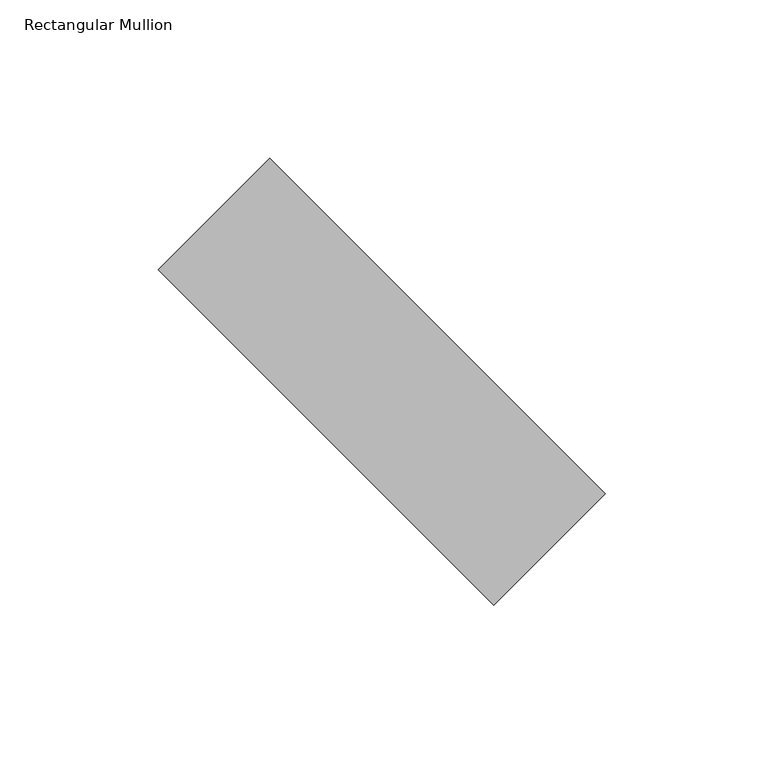
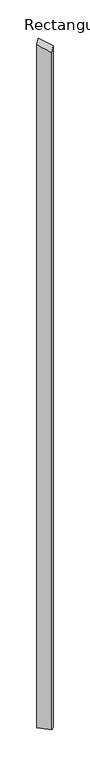
"""IFC4 building model written with IfcOpenShell, lengths in millimetres: member geometry, Rectangular Mullion : tilted mullions."""

from ifc_helpers import new_model, si_unit, origin, place, context, project, spatial, faceted_brep, source, transform, mapped, element, save


def rectangular_mullion_43aaade2(model_context):
    return source(origin(), model_context, "Body", "Brep", [
        faceted_brep([(-35.3553391, 70.7106781, -7999.1801797), (70.7106781, -35.3553391, -7999.1801797), (35.3553391, -70.7106781, -7999.1801797), (-70.7106781, 35.3553391, -7999.1801797), (-70.7106781, 35.3553391, 10.0345933), (-35.3553391, 70.7106781, 55.0781847), (35.3553391, -70.7106781, -55.0781847), (70.7106781, -35.3553391, -10.0345933)], [[[0, 1, 2, 3]], [[4, 5, 0, 3]], [[6, 4, 3, 2]], [[7, 6, 2, 1]], [[5, 7, 1, 0]], [[5, 4, 6, 7]]]),
    ])


if __name__ == "__main__":
    model = new_model("IFC4")
    model_context = context("Model", 3, world=origin())
    ifc_project = project(units=[si_unit("LENGTHUNIT", "METRE", prefix="MILLI")], contexts=[model_context])
    site = spatial("IfcSite", under=ifc_project)
    building = spatial("IfcBuilding", under=site)
    placement = place(None, origin())
    rectangular_mullion_shape = rectangular_mullion_43aaade2(model_context)
    element("IfcMember", 1, ObjectType="Rectangular Mullion : tilted mullions", at=placement, inside=building, context=model_context, shape_type="MappedRepresentation", body=[
        mapped(rectangular_mullion_shape, transform((0.0, 0.0, 0.0), x_axis=(1.0, 0.0, 0.0), y_axis=(0.0, 1.0, 0.0), z_axis=(0.0, 0.0, 1.0))),
    ])
    save(model, "model.ifc")

# Revit data of these elements
# Type "Rectangular Mullion : tilted mullions"
#   built-in parameter 1007304 = 0.492126 (stored number, unit not read)
#   built-in parameter 1007301 = 0.082021 (stored number, unit not read)
#   built-in parameter 1007300 = 0.082021 (stored number, unit not read)
# Element 1 (IfcMember, "Rectangular Mullion : tilted mullions")
#   Materials on its faces: "Aluminum"
# Materials
#   "Aluminum": class "Metal", colour RGB 244 244 244, transparency 0, Description = "Aluminum 6061", Cost = 0
